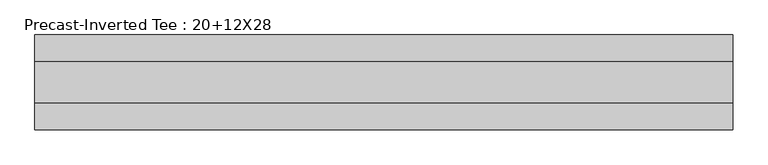
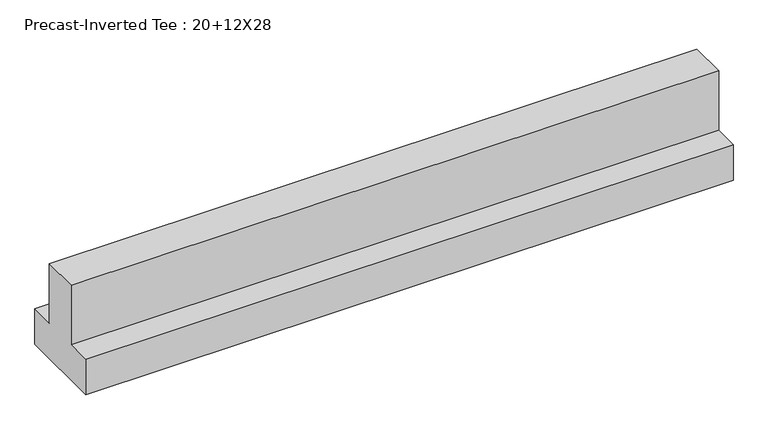
"""IFC4 building model written with IfcOpenShell, lengths in millimetres: beam geometry, Precast-Inverted Tee : 20+12X28."""

from ifc_helpers import new_model, si_unit, frame, origin, place, context, project, spatial, polyline, outline, extrude, source, transform, mapped, element, save


def precast_inverted_tee_20_12x28_0a739a6f(model_context):
    return source(origin(), model_context, "Body", "SweptSolid", [
        extrude(outline(polyline([(355.6, -406.4), (-355.6, -406.4), (-355.6, -101.6), (-152.4, -101.6), (-152.4, 406.4), (152.4, 406.4), (152.4, -101.6), (355.6, -101.6), (355.6, -406.4)])), frame((-2692.4, 0.0, 0.0), z_axis=(1.0, 0.0, 0.0), x_axis=(0.0, 1.0, 0.0)), (0.0, 0.0, 1.0), 5245.1),
    ])


if __name__ == "__main__":
    model = new_model("IFC4")
    model_context = context("Model", 3, world=origin())
    ifc_project = project(units=[si_unit("LENGTHUNIT", "METRE", prefix="MILLI")], contexts=[model_context])
    site = spatial("IfcSite", under=ifc_project)
    building = spatial("IfcBuilding", under=site)
    placement = place(None, origin())
    precast_inverted_tee_20_12x28_shape = precast_inverted_tee_20_12x28_0a739a6f(model_context)
    element("IfcBeam", 1, ObjectType="Precast-Inverted Tee : 20+12X28", at=placement, inside=building, context=model_context, shape_type="MappedRepresentation", body=[
        mapped(precast_inverted_tee_20_12x28_shape, transform((0.0, 0.0, 0.0), x_axis=(1.0, 0.0, 0.0), y_axis=(0.0, 1.0, 0.0), z_axis=(0.0, 0.0, 1.0))),
    ])
    save(model, "model.ifc")

# Revit data of these elements
# Type "Precast-Inverted Tee : 20+12X28"
#   Assembly Code = "B10"
#   Seat = 0' - 8"
#   Length [instance default] = 5' - 0"
#   b = 2' - 4"
#   h = 2' - 8"
#   h1 = 1' - 8"
#   Structural Material [instance default] = Concrete - Precast Concrete - Normal Weight Concrete - 5 ksi
# Element 1 (IfcBeam, "Precast-Inverted Tee : 20+12X28")
#   Length = 17' - 3"
#   Materials on its faces: "Concrete - Precast Concrete - Normal Weight Concrete - 5 ksi"
# Materials
#   "Concrete - Precast Concrete - Normal Weight Concrete - 5 ksi": class "Concrete", colour RGB 198 187 187, transparency 0, Cost = 0
